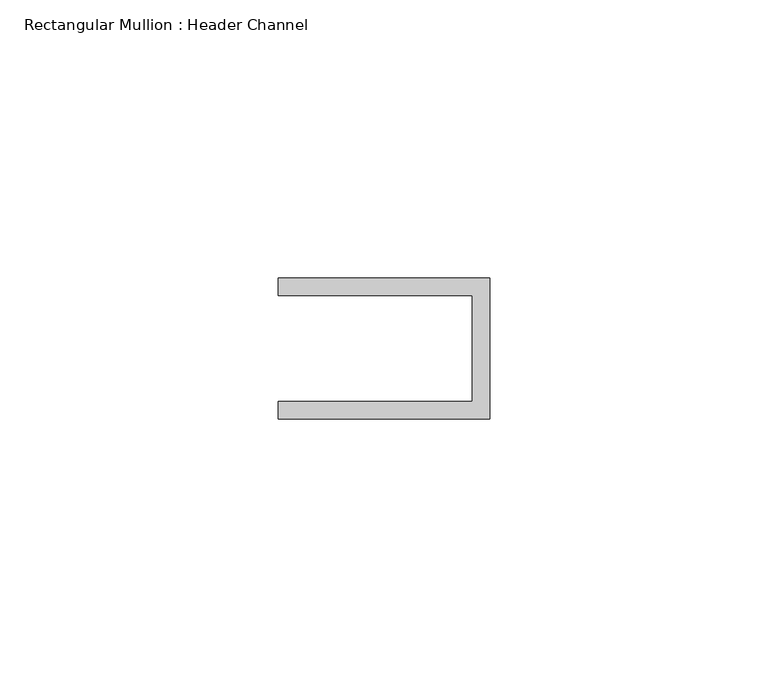
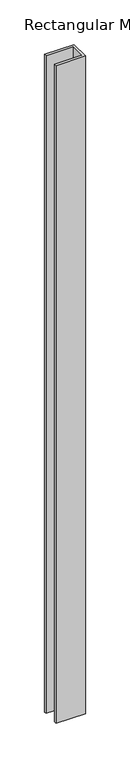
"""IFC4 building model written with IfcOpenShell, lengths in millimetres: member geometry, Rectangular Mullion : Header Channel."""

from ifc_helpers import new_model, si_unit, frame, origin, place, context, project, spatial, polyline, outline, extrude, source, transform, mapped, element, save


def rectangular_mullion_header_channel_139e3a5c(model_context):
    return source(origin(), model_context, "Body", "SweptSolid", [
        extrude(outline(polyline([(0.0, 12.7), (0.0, -12.7), (-38.1, -12.7), (-38.1, -9.525), (-3.175, -9.525), (-3.175, 9.525), (-38.1, 9.525), (-38.1, 12.7), (0.0, 12.7)])), frame((0.0, 0.0, -898.525), z_axis=(0.0, 0.0, 1.0), x_axis=(1.0, 0.0, 0.0)), (0.0, 0.0, 1.0), 898.525),
    ])


if __name__ == "__main__":
    model = new_model("IFC4")
    model_context = context("Model", 3, world=origin())
    ifc_project = project(units=[si_unit("LENGTHUNIT", "METRE", prefix="MILLI")], contexts=[model_context])
    site = spatial("IfcSite", under=ifc_project)
    building = spatial("IfcBuilding", under=site)
    placement = place(None, origin())
    rectangular_mullion_header_channel_shape = rectangular_mullion_header_channel_139e3a5c(model_context)
    element("IfcMember", 1, ObjectType="Rectangular Mullion : Header Channel", at=placement, inside=building, context=model_context, shape_type="MappedRepresentation", body=[
        mapped(rectangular_mullion_header_channel_shape, transform((0.0, 0.0, 0.0), x_axis=(1.0, 0.0, 0.0), y_axis=(0.0, 1.0, 0.0), z_axis=(0.0, 0.0, 1.0))),
    ])
    save(model, "model.ifc")

# Revit data of these elements
# Type "Rectangular Mullion : Header Channel"
#   built-in parameter 1007322 = 0.0833333 (stored number, unit not read)
#   built-in parameter 1007321 = -0.03125 (stored number, unit not read)
#   built-in parameter 1007320 = 0.0416667 (stored number, unit not read)
# Element 1 (IfcMember, "Rectangular Mullion : Header Channel")
#   Materials on its faces: "ALUM"
# Materials
#   "ALUM": class "Generic", colour RGB 157 157 157, transparency 0, Cost = 0
